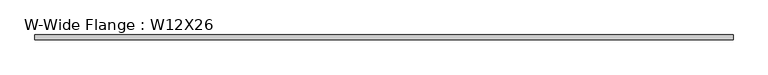
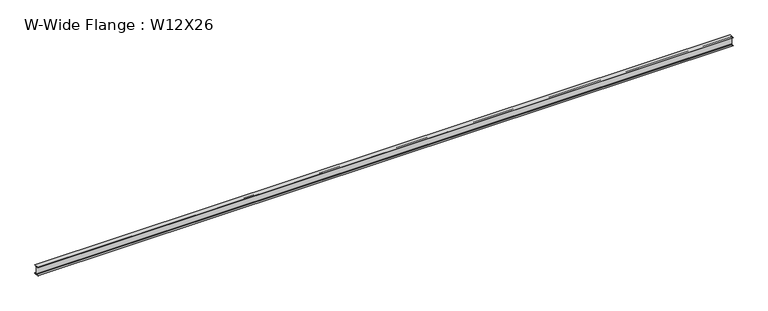
"""IFC4 building model written with IfcOpenShell, lengths in millimetres: beam geometry, W-Wide Flange : W12X26."""

from ifc_helpers import new_model, si_unit, point, frame, frame_2d, origin, place, context, project, spatial, polyline, circle_curve, trimmed, segment, composite_curve, outline, extrude, source, transform, mapped, element, save


def w_wide_flange_w12x26_4eb6bcdb(model_context):
    return source(origin(), model_context, "Body", "SweptSolid", [
        extrude(outline(composite_curve([segment(polyline([(82.4011719, -145.5539063), (82.4011719, -155.178125), (-82.4011719, -155.178125), (-82.4011719, -145.5539063), (-20.2902344, -145.5539063)]), True, "CONTINUOUS"), segment(trimmed(circle_curve(frame_2d((-20.2902344, -128.190625)), 17.3632812), [point((-20.2902344, -145.5539063))], [point((-2.9269531, -128.190625))], True, "CARTESIAN"), True, "CONTINUOUS"), segment(polyline([(-2.9269531, -128.190625), (-2.9269531, 128.190625)]), True, "CONTINUOUS"), segment(trimmed(circle_curve(frame_2d((-20.2902344, 128.190625)), 17.3632812), [point((-2.9269531, 128.190625))], [point((-20.2902344, 145.5539062))], True, "CARTESIAN"), True, "CONTINUOUS"), segment(polyline([(-20.2902344, 145.5539062), (-82.4011719, 145.5539062), (-82.4011719, 155.178125), (82.4011719, 155.178125), (82.4011719, 145.5539062), (20.2902344, 145.5539062)]), True, "CONTINUOUS"), segment(trimmed(circle_curve(frame_2d((20.2902344, 128.190625)), 17.3632812), [point((20.2902344, 145.5539062))], [point((2.9269531, 128.190625))], True, "CARTESIAN"), True, "CONTINUOUS"), segment(polyline([(2.9269531, 128.190625), (2.9269531, -128.190625)]), True, "CONTINUOUS"), segment(trimmed(circle_curve(frame_2d((20.2902344, -128.190625)), 17.3632812), [point((2.9269531, -128.190625))], [point((20.2902344, -145.5539063))], True, "CARTESIAN"), True, "CONTINUOUS"), segment(polyline([(20.2902344, -145.5539063), (82.4011719, -145.5539063)]), True, "CONTINUOUS")], self_intersect=False)), frame((-12158.6625, 0.0, 0.0), z_axis=(1.0, 0.0, 0.0), x_axis=(0.0, 1.0, 0.0)), (0.0, 0.0, 1.0), 24426.8625),
    ])


if __name__ == "__main__":
    model = new_model("IFC4")
    model_context = context("Model", 3, world=origin())
    ifc_project = project(units=[si_unit("LENGTHUNIT", "METRE", prefix="MILLI")], contexts=[model_context])
    site = spatial("IfcSite", under=ifc_project)
    building = spatial("IfcBuilding", under=site)
    placement = place(None, origin())
    w_wide_flange_w12x26_shape = w_wide_flange_w12x26_4eb6bcdb(model_context)
    element("IfcBeam", 1, ObjectType="W-Wide Flange : W12X26", at=placement, inside=building, context=model_context, shape_type="MappedRepresentation", body=[
        mapped(w_wide_flange_w12x26_shape, transform((0.0, 0.0, 0.0), x_axis=(1.0, 0.0, 0.0), y_axis=(0.0, 1.0, 0.0), z_axis=(0.0, 0.0, 1.0))),
    ])
    save(model, "model.ifc")

# Revit data of these elements
# Type "W-Wide Flange : W12X26"
#   Assembly Code = "B10"
#   W = 26
#   Length [instance default] = 5' - 0"
#   bf = 0' - 6 125/256"
#   d = 1' - 0 7/32"
#   k = 0' - 1 1/16"
#   k2 = 0' - 0 175/256"
#   tf = 0' - 0 97/256"
#   tw = 0' - 0 59/256"
#   A = 0.053125 SF
#   Structural Material [instance default] = none
